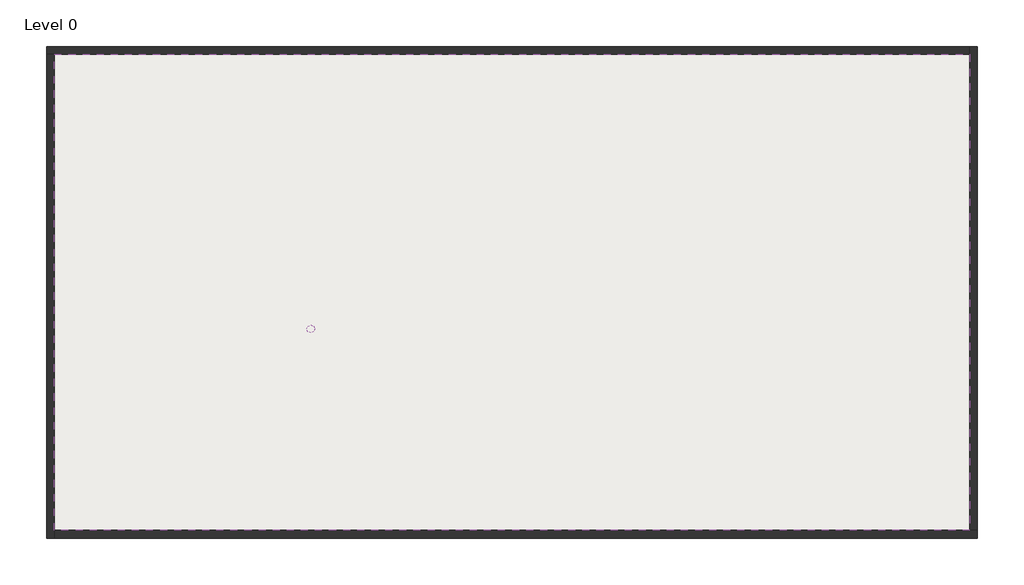
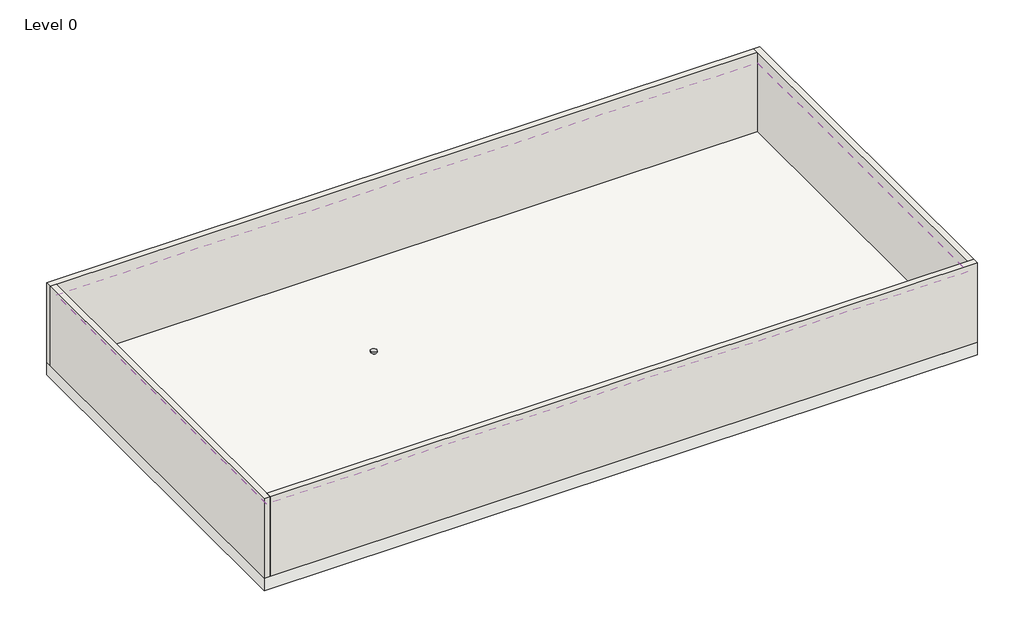
# One storey: 4 walls, 1 covering, 1 electric appliance, 1 slab.
"""IFC4 building model written with IfcOpenShell, lengths in millimetres."""

import ifcopenshell
import ifcopenshell.guid

model = None  # the IFC model being written
_history = None  # IfcOwnerHistory: only IFC2X3 demands one
_inside = {}  # id of a spatial element -> (the spatial element, [elements in it])
_under = {}  # id of a project, library or spatial element -> (it, [spatial elements below it])
_declared = {}  # id of a project -> (the project, [libraries it declares])
_typed = {}  # id of a type object -> (the type object, [elements of that type])
_made_of = {}  # id of a material, layer set ... -> (it, [elements and type objects made of it])


def new_model(schema):
    """Start an empty IFC model of exactly this schema.

    Asked for "IFC4X3", IfcOpenShell would pick the latest addendum, in which some entities
    have other attributes; the version numbers below select the first issue.
    IFC2X3 requires an IfcOwnerHistory on every rooted entity: one is made here for all.
    """
    global model, _history
    if schema == "IFC4X3":
        model = ifcopenshell.file(schema_version=(4, 3, 0, 0))
    else:
        model = ifcopenshell.file(schema=schema)
    _inside.clear()
    _under.clear()
    _declared.clear()
    _typed.clear()
    _made_of.clear()
    _history = None
    if model.schema == "IFC2X3":
        org = make("IfcOrganization", Name="unknown")
        user = make(
            "IfcPersonAndOrganization",
            ThePerson=make("IfcPerson", FamilyName="unknown"),
            TheOrganization=org,
        )
        app = make(
            "IfcApplication",
            ApplicationDeveloper=org,
            Version="unknown",
            ApplicationFullName="unknown",
            ApplicationIdentifier="unknown",
        )
        _history = make(
            "IfcOwnerHistory",
            OwningUser=user,
            OwningApplication=app,
            ChangeAction="ADDED",
            CreationDate=0,
        )
    return model


def make(cls, **values):
    """One entity of the class cls with the attributes given. An attribute that is None is left unset."""
    return model.create_entity(
        cls, **{name: value for name, value in values.items() if value is not None}
    )


def rooted(cls, **values):
    """An entity with a GlobalId (a new one), such as an element, a storey or a relation."""
    return make(cls, GlobalId=ifcopenshell.guid.new(), OwnerHistory=_history, **values)


def si_unit(unit_type, name, prefix=None):
    """IfcSIUnit, for example si_unit("LENGTHUNIT", "METRE", prefix="MILLI")."""
    return make("IfcSIUnit", UnitType=unit_type, Prefix=prefix, Name=name)


def assignment(units):
    """IfcUnitAssignment: the units of a project."""
    return None if units is None else make("IfcUnitAssignment", Units=units)


def point(xyz):
    """IfcCartesianPoint."""
    return None if xyz is None else make("IfcCartesianPoint", Coordinates=xyz)


def direction(xyz):
    """IfcDirection."""
    return None if xyz is None else make("IfcDirection", DirectionRatios=xyz)


def frame(location, z_axis=None, x_axis=None):
    """IfcAxis2Placement3D, a coordinate frame: its origin and axes. An axis left out is left unset."""
    return make(
        "IfcAxis2Placement3D",
        Location=point(location),
        Axis=direction(z_axis),
        RefDirection=direction(x_axis),
    )


def frame_2d(location, x_axis=None):
    """IfcAxis2Placement2D, a coordinate frame in the plane: its origin and x axis."""
    return make(
        "IfcAxis2Placement2D", Location=point(location), RefDirection=direction(x_axis)
    )


def origin():
    """The frame at (0, 0, 0) with its axes left unset."""
    return frame((0.0, 0.0, 0.0))


def origin_with_axes():
    """The frame at (0, 0, 0) with the z axis (0, 0, 1) and the x axis (1, 0, 0) written out."""
    return frame((0.0, 0.0, 0.0), z_axis=(0.0, 0.0, 1.0), x_axis=(1.0, 0.0, 0.0))


def origin_2d():
    """The frame at (0, 0) in the plane with its x axis left unset."""
    return frame_2d((0.0, 0.0))


def place(relative_to, where):
    """IfcLocalPlacement: puts the frame where relative to a parent placement (None: the world)."""
    return make(
        "IfcLocalPlacement", PlacementRelTo=relative_to, RelativePlacement=where
    )


def context(
    kind, dimensions, precision=None, world=None, true_north=None, identifier=None
):
    """IfcGeometricRepresentationContext, for example the 3D "Model" context."""
    return make(
        "IfcGeometricRepresentationContext",
        ContextIdentifier=identifier,
        ContextType=kind,
        CoordinateSpaceDimension=dimensions,
        Precision=precision,
        WorldCoordinateSystem=world,
        TrueNorth=true_north,
    )


def project(units=None, contexts=None):
    """IfcProject with its units and contexts."""
    return rooted(
        "IfcProject",
        Name="project",
        RepresentationContexts=contexts,
        UnitsInContext=assignment(units),
    )


def spatial(cls, under=None, at=None, **own):
    """A site, building, storey or space (cls), placed at a placement, below another one or the project."""
    s = rooted(cls, ObjectPlacement=at, **own)
    if under is not None:
        _under.setdefault(under.id(), (under, []))[1].append(s)
    return s


def polyline(points):
    """IfcPolyline through the points."""
    return make("IfcPolyline", Points=[point(p) for p in points])


def circle_curve(where, radius):
    """IfcCircle in the frame where."""
    return make("IfcCircle", Position=where, Radius=radius)


def trimmed(basis, trim1, trim2, sense, master):
    """IfcTrimmedCurve: the piece of a basis curve between two trims."""
    return make(
        "IfcTrimmedCurve",
        BasisCurve=basis,
        Trim1=trim1,
        Trim2=trim2,
        SenseAgreement=sense,
        MasterRepresentation=master,
    )


def segment(curve, same_sense, transition):
    """IfcCompositeCurveSegment."""
    return make(
        "IfcCompositeCurveSegment",
        Transition=transition,
        SameSense=same_sense,
        ParentCurve=curve,
    )


def composite_curve(segments, self_intersect=None):
    """IfcCompositeCurve: segments joined end to end."""
    return make("IfcCompositeCurve", Segments=segments, SelfIntersect=self_intersect)


def outline(outer, holes=None, kind="AREA"):
    """IfcArbitraryClosedProfileDef: a profile drawn as a closed curve; with holes, ...WithVoids."""
    if holes is None:
        return make("IfcArbitraryClosedProfileDef", ProfileType=kind, OuterCurve=outer)
    return make(
        "IfcArbitraryProfileDefWithVoids",
        ProfileType=kind,
        OuterCurve=outer,
        InnerCurves=holes,
    )


def extrude(swept, where, along, depth):
    """IfcExtrudedAreaSolid: the profile swept, set in the frame where, extruded along a direction by depth."""
    return make(
        "IfcExtrudedAreaSolid",
        SweptArea=swept,
        Position=where,
        ExtrudedDirection=direction(along),
        Depth=depth,
    )


def faces_of(points, faces, orient=None, outer=None):
    """IfcFace entities. A face is a list of loops; a loop is a list of indices into points, from 0.

    orient and outer hold one flag for each loop. By default every Orientation is true, the
    first loop of a face is its IfcFaceOuterBound and the others are IfcFaceBound.
    """
    made = []
    for i, loops in enumerate(faces):
        bounds = []
        for j, loop in enumerate(loops):
            is_outer = j == 0 if outer is None else outer[i][j]
            bounds.append(
                make(
                    "IfcFaceOuterBound" if is_outer else "IfcFaceBound",
                    Bound=make("IfcPolyLoop", Polygon=[points[k] for k in loop]),
                    Orientation=True if orient is None else orient[i][j],
                )
            )
        made.append(make("IfcFace", Bounds=bounds))
    return made


def faceted_brep(points, faces, orient=None, outer=None, voids=None):
    """IfcFacetedBrep: a solid bounded by flat faces; with voids (closed shells), ...WithVoids."""
    shared = [point(p) for p in points]
    hull = make("IfcClosedShell", CfsFaces=faces_of(shared, faces, orient, outer))
    if voids is None:
        return make("IfcFacetedBrep", Outer=hull)
    return make(
        "IfcFacetedBrepWithVoids",
        Outer=hull,
        Voids=[
            make(cls, CfsFaces=faces_of(shared, fs, o, b)) for cls, fs, o, b in voids
        ],
    )


def shape(context_of_items, identifier, shape_type, items):
    """IfcShapeRepresentation: the items that make up one representation, for example the "Body"."""
    return make(
        "IfcShapeRepresentation",
        ContextOfItems=context_of_items,
        RepresentationIdentifier=identifier,
        RepresentationType=shape_type,
        Items=items,
    )


def source(mapping_origin, context_of_items, identifier, shape_type, items):
    """IfcRepresentationMap: a shape defined once, which mapped items show again and again."""
    return make(
        "IfcRepresentationMap",
        MappingOrigin=mapping_origin,
        MappedRepresentation=shape(context_of_items, identifier, shape_type, items),
    )


def transform(
    local_origin,
    x_axis=None,
    y_axis=None,
    z_axis=None,
    scale=None,
    scale2=None,
    scale3=None,
    uniform=True,
):
    """IfcCartesianTransformationOperator3D, or its non-uniform kind. x_axis, y_axis, z_axis: its Axis1, 2, 3."""
    if uniform:
        return make(
            "IfcCartesianTransformationOperator3D",
            Axis1=direction(x_axis),
            Axis2=direction(y_axis),
            LocalOrigin=point(local_origin),
            Scale=scale,
            Axis3=direction(z_axis),
        )
    return make(
        "IfcCartesianTransformationOperator3DnonUniform",
        Axis1=direction(x_axis),
        Axis2=direction(y_axis),
        LocalOrigin=point(local_origin),
        Scale=scale,
        Axis3=direction(z_axis),
        Scale2=scale2,
        Scale3=scale3,
    )


def mapped(mapping_source, mapping_target):
    """IfcMappedItem: shows the shape of a source again, moved by a transform."""
    return make(
        "IfcMappedItem", MappingSource=mapping_source, MappingTarget=mapping_target
    )


def made_of(thing, what):
    """Note that an element or type object is made of a material, layer set ...; save() writes the relation."""
    if what is not None:
        _made_of.setdefault(what.id(), (what, []))[1].append(thing)
    return thing


def element(
    cls,
    number,
    at=None,
    inside=None,
    cuts=None,
    type_object=None,
    material=None,
    context=None,
    identifier="Body",
    shape_type=None,
    held_by="IfcProductDefinitionShape",
    body=None,
    shapes=None,
    **own,
):
    """One element of the class cls, such as IfcWall. Its Tag is "e" and its number.

    at: its placement. inside: the storey or other place that contains it. cuts: it is an
    opening in that element (IfcRelVoidsElement). A single representation is given by context,
    identifier, shape_type and body (its items); several are given by shapes. held_by: the class
    of the entity that holds the representations. save() writes the other relations.
    """
    e = rooted(cls, Tag="e%d" % number, ObjectPlacement=at, **own)
    if body is not None:
        shapes = [shape(context, identifier, shape_type, body)]
    if shapes is not None:
        e.Representation = make(held_by, Representations=shapes)
    if inside is not None:
        _inside.setdefault(inside.id(), (inside, []))[1].append(e)
    if cuts is not None:
        rooted(
            "IfcRelVoidsElement", RelatingBuildingElement=cuts, RelatedOpeningElement=e
        )
    if type_object is not None:
        _typed.setdefault(type_object.id(), (type_object, []))[1].append(e)
    return made_of(e, material)


def aggregate(whole, parts):
    """IfcRelAggregates: a whole, such as a stair, and the parts it consists of."""
    return rooted("IfcRelAggregates", RelatingObject=whole, RelatedObjects=parts)


def save(model, path):
    """Write the relations noted so far, then the file.

    IfcRelAggregates (storeys below a building ...), IfcRelContainedInSpatialStructure (elements
    in a storey), IfcRelDefinesByType, IfcRelAssociatesMaterial and IfcRelDeclares: one each for
    every whole, place, type object, material and project.
    """
    for whole, parts in _under.values():
        aggregate(whole, parts)
    for where, things in _inside.values():
        rooted(
            "IfcRelContainedInSpatialStructure",
            RelatedElements=things,
            RelatingStructure=where,
        )
    for kind, things in _typed.values():
        rooted("IfcRelDefinesByType", RelatedObjects=things, RelatingType=kind)
    for what, things in _made_of.values():
        rooted("IfcRelAssociatesMaterial", RelatedObjects=things, RelatingMaterial=what)
    for by, libraries in _declared.values():
        rooted("IfcRelDeclares", RelatingContext=by, RelatedDefinitions=libraries)
    model.write(path)


def electric_appliance_a5c8b711(model_context):
    return source(origin(), model_context, "Body", "SweptSolid", [
        extrude(outline(composite_curve([segment(trimmed(circle_curve(origin_2d(), 10.0), [point((-10.0, 0.0))], [point((10.0, 0.0))], False, "CARTESIAN"), True, "CONTINUOUS"), segment(trimmed(circle_curve(origin_2d(), 10.0), [point((10.0, 0.0))], [point((-10.0, 0.0))], False, "CARTESIAN"), True, "CONTINUOUS")], self_intersect=False)), frame((0.0, 0.0, 50.0), z_axis=(0.0, 0.0, 1.0), x_axis=(1.0, 0.0, 0.0)), (0.0, 0.0, 1.0), 81.4052538),
        extrude(outline(composite_curve([segment(trimmed(circle_curve(origin_2d(), 110.0), [point((-110.0, 0.0))], [point((110.0, 0.0))], False, "CARTESIAN"), True, "CONTINUOUS"), segment(trimmed(circle_curve(origin_2d(), 110.0), [point((110.0, 0.0))], [point((-110.0, 0.0))], False, "CARTESIAN"), True, "CONTINUOUS")], self_intersect=False)), origin_with_axes(), (0.0, 0.0, 1.0), 50.0),
    ])


model = new_model("IFC4")

# Units and contexts
model_context = context("Model", 3, world=origin())
ifc_project = project(units=[si_unit("LENGTHUNIT", "METRE", prefix="MILLI")], contexts=[model_context])

# Site, building, storey
site = spatial("IfcSite", under=ifc_project)
building = spatial("IfcBuilding", under=site)
storey = spatial("IfcBuildingStorey", under=building, Name="Level 0", Elevation=0.0)

# Covering
placement = place(None, origin())
element("IfcCovering", 1, ObjectType="Plain", at=placement, inside=storey, context=model_context, shape_type="SweptSolid", body=[
    extrude(outline(polyline([(-6728.9458796, 5967.5463282), (18271.0541204, 5967.5463282), (18271.0541204, -7032.4536718), (-6728.9458796, -7032.4536718), (-6728.9458796, 5967.5463282)])), frame((0.0, 0.0, 2600.0), z_axis=(0.0, 0.0, 1.0), x_axis=(1.0, 0.0, 0.0)), (0.0, 0.0, 1.0), 57.0),
])

# Electric appliance
electric_appliance_shape = electric_appliance_a5c8b711(model_context)
element("IfcElectricAppliance", 2, ObjectType="Wifi Access Point : Wifi Access Point", at=placement, inside=storey, context=model_context, shape_type="MappedRepresentation", body=[
    mapped(electric_appliance_shape, transform((271.0541204, -1532.4536718, 2600.0), x_axis=(1.0, 0.0, 0.0), y_axis=(0.0, -1.0, 0.0), z_axis=(0.0, 0.0, -1.0))),
])

# Slab
element("IfcSlab", 3, ObjectType="Floor-Grnd-Susp_65Scr-80Ins-100Blk-75PC", at=placement, inside=storey, context=model_context, shape_type="SweptSolid", body=[
    extrude(outline(polyline([(18486.0541204, 6182.5463282), (18486.0541204, -7247.4536718), (-6943.9458796, -7247.4536718), (-6943.9458796, 6182.5463282), (18486.0541204, 6182.5463282)])), frame((0.0, 0.0, -470.0), z_axis=(0.0, 0.0, 1.0), x_axis=(1.0, 0.0, 0.0)), (0.0, 0.0, 1.0), 470.0),
])

# Walls
element("IfcWall", 4, ObjectType="Wall-Ext_215Bwk", at=placement, inside=storey, context=model_context, shape_type="Brep", body=[
    faceted_brep([(-6943.9458796, 5967.5463282, 0.0), (-6728.9458796, 5967.5463282, 0.0), (18271.0541204, 5967.5463282, 0.0), (18271.0541204, 5967.5463282, 3000.0), (-6728.9458796, 5967.5463282, 3000.0), (-6943.9458796, 5967.5463282, 3000.0), (-6943.9458796, 6182.5463282, 0.0), (-6943.9458796, 6182.5463282, 3000.0), (18271.0541204, 6182.5463282, 3000.0), (18271.0541204, 6182.5463282, 0.0)], [[[0, 1, 2, 3, 4, 5]], [[6, 7, 8, 9]], [[2, 1, 0, 6, 9]], [[5, 4, 3, 8, 7]], [[0, 5, 7, 6]], [[3, 2, 9, 8]]]),
])
element("IfcWall", 5, ObjectType="Wall-Ext_215Bwk", at=placement, inside=storey, context=model_context, shape_type="Brep", body=[
    faceted_brep([(-6728.9458796, -7247.4536718, 0.0), (-6728.9458796, -7032.4536718, 0.0), (-6728.9458796, 5967.5463282, 0.0), (-6728.9458796, 5967.5463282, 3000.0), (-6728.9458796, -7032.4536718, 3000.0), (-6728.9458796, -7247.4536718, 3000.0), (-6943.9458796, -7247.4536718, 0.0), (-6943.9458796, -7247.4536718, 3000.0), (-6943.9458796, 5967.5463282, 3000.0), (-6943.9458796, 5967.5463282, 0.0)], [[[0, 1, 2, 3, 4, 5]], [[6, 7, 8, 9]], [[2, 1, 0, 6, 9]], [[5, 4, 3, 8, 7]], [[0, 5, 7, 6]], [[3, 2, 9, 8]]]),
])
element("IfcWall", 6, ObjectType="Wall-Ext_215Bwk", at=placement, inside=storey, context=model_context, shape_type="Brep", body=[
    faceted_brep([(18486.0541204, -7032.4536718, 0.0), (18271.0541204, -7032.4536718, 0.0), (-6728.9458796, -7032.4536718, 0.0), (-6728.9458796, -7032.4536718, 3000.0), (18271.0541204, -7032.4536718, 3000.0), (18486.0541204, -7032.4536718, 3000.0), (18486.0541204, -7247.4536718, 0.0), (18486.0541204, -7247.4536718, 3000.0), (-6728.9458796, -7247.4536718, 3000.0), (-6728.9458796, -7247.4536718, 0.0)], [[[0, 1, 2, 3, 4, 5]], [[6, 7, 8, 9]], [[2, 1, 0, 6, 9]], [[5, 4, 3, 8, 7]], [[0, 5, 7, 6]], [[3, 2, 9, 8]]]),
])
element("IfcWall", 7, ObjectType="Wall-Ext_215Bwk", at=placement, inside=storey, context=model_context, shape_type="Brep", body=[
    faceted_brep([(18271.0541204, 6182.5463282, 0.0), (18271.0541204, 5967.5463282, 0.0), (18271.0541204, -7032.4536718, 0.0), (18271.0541204, -7032.4536718, 3000.0), (18271.0541204, 5967.5463282, 3000.0), (18271.0541204, 6182.5463282, 3000.0), (18486.0541204, 6182.5463282, 0.0), (18486.0541204, 6182.5463282, 3000.0), (18486.0541204, -7032.4536718, 3000.0), (18486.0541204, -7032.4536718, 0.0)], [[[0, 1, 2, 3, 4, 5]], [[6, 7, 8, 9]], [[2, 1, 0, 6, 9]], [[5, 4, 3, 8, 7]], [[0, 5, 7, 6]], [[3, 2, 9, 8]]]),
])

save(model, "model.ifc")

# Revit data of these elements
# Project information
#   Project Issue Date = "Issue Date"
#   Project Status = "Project Status"
#   Client Name = "Owner"
#   Project Address = "Enter address here"
#   Project Name = "Project Name"
#   Project Number = "Project Number"
# Type "Plain"
#   Keynote = "K40"
#   built-in parameter 1002203 = 1 (stored number, unit not read)
#   built-in parameter 1002202 = 1 (stored number, unit not read)
#   Layers, outside or top first: 0.045 m "Metal Stud Layer" (function 1); 0.012 m "Gypsum Wall Board" (function 1)
# Type "Wifi Access Point : Wifi Access Point"
#   Default Elevation = 1.2 m
# Type "Floor-Grnd-Susp_65Scr-80Ins-100Blk-75PC"
#   Keynote = "E60/130"
#   Function = 0
#   Layers, outside or top first: 0.065 m "Concrete, Sand/Cement Screed" (function 4); 0 m "Vapor Retarder" (function 100); 0.08 m "Rigid insulation" (function 3); 0.15 m "Air" (function 3); 0 m "Damp-proofing" (function 100); 0.1 m "Concrete Masonry, Floor Block" (function 1); 0.075 m "Concrete, Precast" (function 1)
# Type "Wall-Ext_215Bwk"
#   Keynote = "F10"
#   Layers, outside or top first: 0.215 m "Brick, Common" (function 1)
# Element 1 (IfcCovering, "Plain")
#   Height Offset From Level = 2.6 m
#   Phase Created = New Construction
#   Materials on its faces: "Gypsum Wall Board", "Metal Stud Layer"
# Element 2 (IfcElectricAppliance, "Wifi Access Point : Wifi Access Point")
#   Mark = "1"
#   Phase Created = New Construction
# Element 3 (IfcSlab, "Floor-Grnd-Susp_65Scr-80Ins-100Blk-75PC")
#   Height Offset From Level = 0 m
#   Phase Created = New Construction
#   Materials on its faces: "Concrete, Precast", "Concrete, Sand/Cement Screed"
# Elements 4, 5, 6, 7 (IfcWall, "Wall-Ext_215Bwk")
#   Top Offset = 0 m
#   Base Offset = 0 m
#   Unconnected Height = 3 m
#   wall height = 3 m
#   Phase Created = New Construction
#   Base Constraint = Level 0
#   Materials on its faces: "Brick, Common"
# Materials
#   "Metal Stud Layer": class "Metal", colour RGB 127 127 127, transparency 0, Description = "Light gauge steel framing, thermal air layer", Cost = 0
#   "Gypsum Wall Board": class "Generic", colour RGB 249 249 249, transparency 0, Description = "Gypsum Wall Board", Cost = 0
#   "Concrete, Sand/Cement Screed": class "Concrete", colour RGB 127 127 127, transparency 0, Description = "Concrete slab topping", Cost = 0
#   "Vapor Retarder": class "Generic", colour RGB 120 120 120, transparency 0, Description = "Polyethylene film membrane", Cost = 0
#   "Rigid insulation": class "Generic", colour RGB 127 127 127, transparency 0, Description = "Rigid foam insulation board", Cost = 0
#   "Air": class "Gas", colour RGB 255 255 255, transparency 0, Description = "Air", Cost = 0
#   "Damp-proofing": class "Generic", colour RGB 127 127 127, transparency 0, Description = "Damp-proofing", Cost = 0
#   "Concrete Masonry, Floor Block": class "Concrete", colour RGB 181 181 181, transparency 0, Description = "physical material", Cost = 0
#   "Concrete, Precast": class "Concrete", colour RGB 192 192 192, transparency 0, Description = "Precast concrete", Cost = 0
#   "Brick, Common": class "Masonry", colour RGB 170 100 105, transparency 0, Description = "Common brick", Cost = 0
